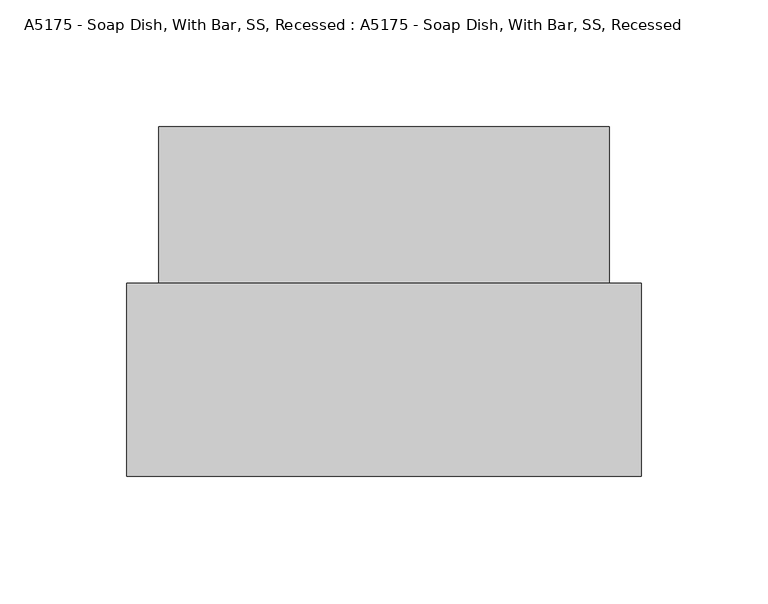
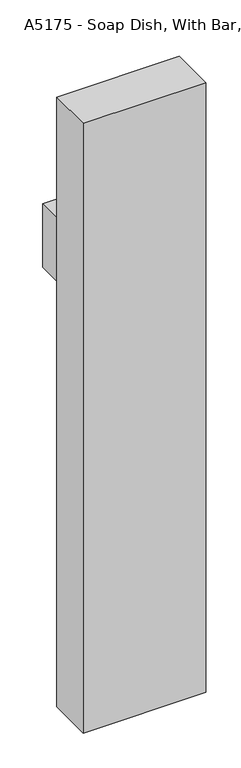
"""IFC4 building model written with IfcOpenShell, lengths in millimetres: proxy geometry, A5175 - Soap Dish, With Bar, SS, Recessed : A5175 - Soap Dish, With Bar, SS, Recessed."""

from ifc_helpers import new_model, si_unit, frame, origin, place, context, project, spatial, circle_curve, ellipse_curve, faceted_brep, source, transform, mapped, element, save
from ifc_brep_helpers import plane_surface, cylinder_surface, advanced_brep


def a5175_soap_dish_with_bar_ss_recessed_a5175_soap_dish_with_60321abb(model_context):
    return source(origin(), model_context, "Body", "SolidModel", [
        advanced_brep(
        [(-73.0659295, -74.6125, 762.0315243), (-79.4157151, -74.6125, 762.0315243), (-79.4157151, -90.4873928, 762.0315243), (-73.0659295, -84.1376072, 762.0315243), (79.3340705, -90.4873928, 762.0315243), (72.9842849, -84.1376072, 762.0315243), (72.9842849, -74.6125, 762.0315243), (79.3340705, -74.6125, 762.0315243)],
        [
            (0, 1, circle_curve(frame((-76.2408223, -74.6125, 762.0315243), z_axis=(0.0, 1.0, 0.0), x_axis=(-1.0, 0.0, 0.0)), 3.1748928)),
            (1, 0, circle_curve(frame((-76.2408223, -74.6125, 762.0315243), z_axis=(0.0, 1.0, 0.0), x_axis=(-1.0, 0.0, 0.0)), 3.1748928)),
            (1, 2),
            (2, 3, ellipse_curve(frame((-76.2408223, -87.3125, 762.0315243), z_axis=(-0.7071067811865475, 0.7071067811865475, 0.0), x_axis=(0.7071067811865474, 0.7071067811865476, 0.0)), 4.4899765, 3.1748928)),
            (3, 0),
            (3, 2, ellipse_curve(frame((-76.2408223, -87.3125, 762.0315243), z_axis=(-0.7071067811865475, 0.7071067811865475, 0.0), x_axis=(0.7071067811865474, 0.7071067811865476, 0.0)), 4.4899765, 3.1748928)),
            (2, 4),
            (4, 5, ellipse_curve(frame((76.1591777, -87.3125, 762.0315243), z_axis=(-0.7071067811865475, -0.7071067811865475, 0.0), x_axis=(-0.7071067811865476, 0.7071067811865474, 0.0)), 4.4899765, 3.1748928)),
            (5, 3),
            (5, 4, ellipse_curve(frame((76.1591777, -87.3125, 762.0315243), z_axis=(-0.7071067811865475, -0.7071067811865475, 0.0), x_axis=(-0.7071067811865476, 0.7071067811865474, 0.0)), 4.4899765, 3.1748928)),
            (6, 7, circle_curve(frame((76.1591777, -74.6125, 762.0315243), z_axis=(0.0, 1.0, 0.0), x_axis=(1.0, 0.0, 0.0)), 3.1748928)),
            (7, 6, circle_curve(frame((76.1591777, -74.6125, 762.0315243), z_axis=(0.0, 1.0, 0.0), x_axis=(1.0, 0.0, 0.0)), 3.1748928)),
            (4, 7),
            (6, 5),
        ],
        [
            plane_surface(frame((-76.2408223, -74.6125, 762.0315243), z_axis=(0.0, 1.0, 0.0), x_axis=(0.0, 0.0, 1.0))),
            cylinder_surface(frame((-76.2408223, -74.6125, 762.0315243), z_axis=(0.0, 1.0, 0.0), x_axis=(-1.0, 0.0, 0.0)), 3.1748928),
            cylinder_surface(frame((-76.2408223, -87.3125, 762.0315243), z_axis=(-1.0, 0.0, 0.0), x_axis=(0.0, -1.0, 0.0)), 3.1748928),
            plane_surface(frame((76.1591777, -74.6125, 762.0315243), z_axis=(0.0, 1.0, 0.0), x_axis=(0.0, 0.0, 1.0))),
            cylinder_surface(frame((76.1591777, -87.3125, 762.0315243), z_axis=(0.0, -1.0, 0.0), x_axis=(1.0, 0.0, 0.0)), 3.1748928),
        ],
        [
            (0, [[1, 2]]),
            (1, [[3, 4, 5, -2]]),
            (1, [[-5, 6, -3, -1]]),
            (2, [[7, 8, 9, -4]]),
            (2, [[-9, 10, -7, -6]]),
            (3, [[11, 12]]),
            (4, [[13, -11, 14, -8]]),
            (4, [[-14, -12, -13, -10]]),
        ],
    ),
        faceted_brep([(-69.85, -13.796456, 817.5393161), (-69.85, -88.9, 817.5393161), (-69.85, -88.9, 741.3393161), (-69.85, -13.796456, 741.3393161), (69.85, -13.796456, 817.5393161), (69.85, -88.9, 817.5393161), (69.85, -13.796456, 741.3393161), (69.85, -88.9, 741.3393161), (-88.9, -88.9, 726.6299448), (88.9, -88.9, 726.6299448), (88.9, -88.9, 838.2), (-88.9, -88.9, 838.2), (-88.9, 0.0, 726.6299448), (-88.9, 0.0, 838.2), (88.9, 0.0, 838.2), (88.9, 0.0, 726.6299448)], [[[0, 1, 2, 3]], [[4, 5, 1, 0]], [[6, 7, 5, 4]], [[3, 2, 7, 6]], [[8, 9, 10, 11], [1, 5, 7, 2]], [[12, 13, 14, 15]], [[11, 13, 12, 8]], [[10, 14, 13, 11]], [[9, 15, 14, 10]], [[8, 12, 15, 9]], [[3, 6, 4, 0]]]),
        faceted_brep([(101.6, -138.1125, 1066.8), (101.6, -61.9125, 1066.8), (-101.6, -61.9125, 1066.8), (-101.6, -138.1125, 1066.8), (101.6, -138.1125, 0.0), (-101.6, -138.1125, 0.0), (-101.6, -61.9125, 0.0), (101.6, -61.9125, 0.0), (-69.85, -61.9125, 741.3393161), (69.85, -61.9125, 741.3393161), (69.85, -61.9125, 817.5393161), (-69.85, -61.9125, 817.5393161), (-69.85, -88.9, 741.3393161), (-69.85, -88.9, 817.5393161), (69.85, -88.9, 817.5393161), (69.85, -88.9, 741.3393161)], [[[0, 1, 2, 3]], [[4, 5, 6, 7]], [[3, 5, 4, 0]], [[2, 6, 5, 3]], [[1, 7, 6, 2], [8, 9, 10, 11]], [[0, 4, 7, 1]], [[12, 13, 14, 15]], [[12, 8, 11, 13]], [[13, 11, 10, 14]], [[14, 10, 9, 15]], [[15, 9, 8, 12]]]),
    ])


if __name__ == "__main__":
    model = new_model("IFC4")
    model_context = context("Model", 3, world=origin())
    ifc_project = project(units=[si_unit("LENGTHUNIT", "METRE", prefix="MILLI")], contexts=[model_context])
    site = spatial("IfcSite", under=ifc_project)
    building = spatial("IfcBuilding", under=site)
    placement = place(None, origin())
    a5175_soap_dish_with_bar_ss_recessed_a5175_soap_dish_with_shape = a5175_soap_dish_with_bar_ss_recessed_a5175_soap_dish_with_60321abb(model_context)
    element("IfcBuildingElementProxy", 1, Name="A5175 - Soap Dish, With Bar, SS, Recessed : A5175 - Soap Dish, With Bar, SS, Recessed", ObjectType="A5175 - Soap Dish, With Bar, SS, Recessed : A5175 - Soap Dish, With Bar, SS, Recessed", at=placement, inside=building, context=model_context, shape_type="MappedRepresentation", body=[
        mapped(a5175_soap_dish_with_bar_ss_recessed_a5175_soap_dish_with_shape, transform((0.0, 0.0, 0.0), x_axis=(1.0, 0.0, 0.0), y_axis=(0.0, 1.0, 0.0), z_axis=(0.0, 0.0, 1.0))),
    ])
    save(model, "model.ifc")

# Revit data of these elements
# Type "A5175 - Soap Dish, With Bar, SS, Recessed : A5175 - Soap Dish, With Bar, SS, Recessed"
#   Watts2 = "0"
#   Watts1 = "0"
#   Unit_Issue = "EA"
#   UTIL_6_Misc = "-"
#   UTIL_5_NonMedGas = "-"
#   UTIL_4_MiscGas = "-"
#   UTIL_3_MedGas = "-"
#   UTIL_2_Elec = "-"
#   UTIL_1_WaterDrain = "-"
#   Nomenclature = "Soap Dish, With Bar, SS, Recessed"
#   NSN = "4510"
#   Location [instance default] = ""
#   JSN = "A5175"
#   Fund_Source_VA = "-"
#   Fund_Source_Navy = "-"
#   Fund_Source_Army = "-"
#   Fund_Source_AF = "-"
#   ELEC_Volts2 = "0"
#   ELEC_Volts1 = "0"
#   ELEC_Phase2 = "0"
#   ELEC_Phase1 = "0"
#   ELEC_HertzSwitch = "0"
#   ELEC_HertzDependent = "0"
#   ELEC_Hertz = "0"
#   ELEC_Amps2 = "0"
#   ELEC_Amps1 = "0"
#   DetailDescription = "A recessed mounted, satin finish stainless steel, soap dish with bar. Soap dish furnished with retaining lip and mounting clamp for installation in stud walls or countertop aprons. For general purpose use in shower stalls or at bathtub locations."
#   CAT_VA = "A"
#   CAT_Navy = "A"
#   CAT_IHS = "-"
#   CAT_Army = "A"
#   CAT_AF = "A"
#   BTUperhour = "0"
#   Weight_IP = 1
#   DIM_Width_IP = 0' - 8"
#   DIM_Height_IP = 3' - 6"
#   DIM_Depth_IP = 0' - 3"
# Element 1 (IfcBuildingElementProxy, "A5175 - Soap Dish, With Bar, SS, Recessed : A5175 - Soap Dish, With Bar, SS, Recessed")
#   Location = "TLTS2"
#   Materials on its faces: "EquipSpace"
# Materials
#   "EquipSpace": class "Unassigned", colour RGB 221 217 195, transparency 0.5
